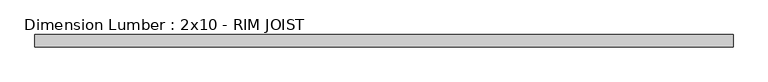
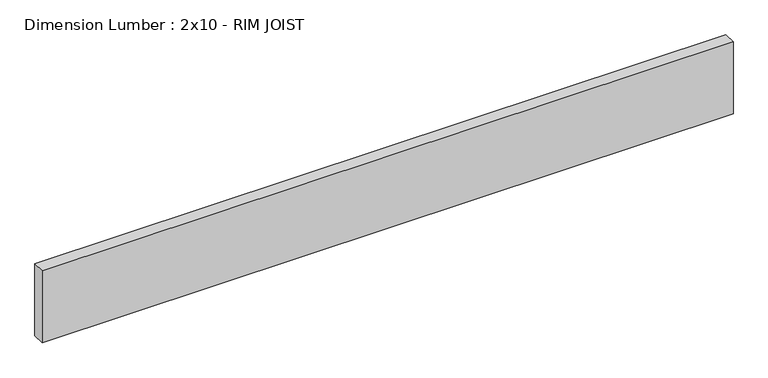
"""IFC4 building model written with IfcOpenShell, lengths in millimetres: beam geometry, Dimension Lumber : 2x10 - RIM JOIST."""

import ifcopenshell
import ifcopenshell.guid

model = None  # the IFC model being written
_history = None  # IfcOwnerHistory: only IFC2X3 demands one
_inside = {}  # id of a spatial element -> (the spatial element, [elements in it])
_under = {}  # id of a project, library or spatial element -> (it, [spatial elements below it])
_declared = {}  # id of a project -> (the project, [libraries it declares])
_typed = {}  # id of a type object -> (the type object, [elements of that type])
_made_of = {}  # id of a material, layer set ... -> (it, [elements and type objects made of it])


def new_model(schema):
    """Start an empty IFC model of exactly this schema.

    Asked for "IFC4X3", IfcOpenShell would pick the latest addendum, in which some entities
    have other attributes; the version numbers below select the first issue.
    IFC2X3 requires an IfcOwnerHistory on every rooted entity: one is made here for all.
    """
    global model, _history
    if schema == "IFC4X3":
        model = ifcopenshell.file(schema_version=(4, 3, 0, 0))
    else:
        model = ifcopenshell.file(schema=schema)
    _inside.clear()
    _under.clear()
    _declared.clear()
    _typed.clear()
    _made_of.clear()
    _history = None
    if model.schema == "IFC2X3":
        org = make("IfcOrganization", Name="unknown")
        user = make(
            "IfcPersonAndOrganization",
            ThePerson=make("IfcPerson", FamilyName="unknown"),
            TheOrganization=org,
        )
        app = make(
            "IfcApplication",
            ApplicationDeveloper=org,
            Version="unknown",
            ApplicationFullName="unknown",
            ApplicationIdentifier="unknown",
        )
        _history = make(
            "IfcOwnerHistory",
            OwningUser=user,
            OwningApplication=app,
            ChangeAction="ADDED",
            CreationDate=0,
        )
    return model


def make(cls, **values):
    """One entity of the class cls with the attributes given. An attribute that is None is left unset."""
    return model.create_entity(
        cls, **{name: value for name, value in values.items() if value is not None}
    )


def rooted(cls, **values):
    """An entity with a GlobalId (a new one), such as an element, a storey or a relation."""
    return make(cls, GlobalId=ifcopenshell.guid.new(), OwnerHistory=_history, **values)


def si_unit(unit_type, name, prefix=None):
    """IfcSIUnit, for example si_unit("LENGTHUNIT", "METRE", prefix="MILLI")."""
    return make("IfcSIUnit", UnitType=unit_type, Prefix=prefix, Name=name)


def assignment(units):
    """IfcUnitAssignment: the units of a project."""
    return None if units is None else make("IfcUnitAssignment", Units=units)


def point(xyz):
    """IfcCartesianPoint."""
    return None if xyz is None else make("IfcCartesianPoint", Coordinates=xyz)


def direction(xyz):
    """IfcDirection."""
    return None if xyz is None else make("IfcDirection", DirectionRatios=xyz)


def frame(location, z_axis=None, x_axis=None):
    """IfcAxis2Placement3D, a coordinate frame: its origin and axes. An axis left out is left unset."""
    return make(
        "IfcAxis2Placement3D",
        Location=point(location),
        Axis=direction(z_axis),
        RefDirection=direction(x_axis),
    )


def origin():
    """The frame at (0, 0, 0) with its axes left unset."""
    return frame((0.0, 0.0, 0.0))


def place(relative_to, where):
    """IfcLocalPlacement: puts the frame where relative to a parent placement (None: the world)."""
    return make(
        "IfcLocalPlacement", PlacementRelTo=relative_to, RelativePlacement=where
    )


def context(
    kind, dimensions, precision=None, world=None, true_north=None, identifier=None
):
    """IfcGeometricRepresentationContext, for example the 3D "Model" context."""
    return make(
        "IfcGeometricRepresentationContext",
        ContextIdentifier=identifier,
        ContextType=kind,
        CoordinateSpaceDimension=dimensions,
        Precision=precision,
        WorldCoordinateSystem=world,
        TrueNorth=true_north,
    )


def project(units=None, contexts=None):
    """IfcProject with its units and contexts."""
    return rooted(
        "IfcProject",
        Name="project",
        RepresentationContexts=contexts,
        UnitsInContext=assignment(units),
    )


def spatial(cls, under=None, at=None, **own):
    """A site, building, storey or space (cls), placed at a placement, below another one or the project."""
    s = rooted(cls, ObjectPlacement=at, **own)
    if under is not None:
        _under.setdefault(under.id(), (under, []))[1].append(s)
    return s


def polyline(points):
    """IfcPolyline through the points."""
    return make("IfcPolyline", Points=[point(p) for p in points])


def outline(outer, holes=None, kind="AREA"):
    """IfcArbitraryClosedProfileDef: a profile drawn as a closed curve; with holes, ...WithVoids."""
    if holes is None:
        return make("IfcArbitraryClosedProfileDef", ProfileType=kind, OuterCurve=outer)
    return make(
        "IfcArbitraryProfileDefWithVoids",
        ProfileType=kind,
        OuterCurve=outer,
        InnerCurves=holes,
    )


def extrude(swept, where, along, depth):
    """IfcExtrudedAreaSolid: the profile swept, set in the frame where, extruded along a direction by depth."""
    return make(
        "IfcExtrudedAreaSolid",
        SweptArea=swept,
        Position=where,
        ExtrudedDirection=direction(along),
        Depth=depth,
    )


def shape(context_of_items, identifier, shape_type, items):
    """IfcShapeRepresentation: the items that make up one representation, for example the "Body"."""
    return make(
        "IfcShapeRepresentation",
        ContextOfItems=context_of_items,
        RepresentationIdentifier=identifier,
        RepresentationType=shape_type,
        Items=items,
    )


def source(mapping_origin, context_of_items, identifier, shape_type, items):
    """IfcRepresentationMap: a shape defined once, which mapped items show again and again."""
    return make(
        "IfcRepresentationMap",
        MappingOrigin=mapping_origin,
        MappedRepresentation=shape(context_of_items, identifier, shape_type, items),
    )


def transform(
    local_origin,
    x_axis=None,
    y_axis=None,
    z_axis=None,
    scale=None,
    scale2=None,
    scale3=None,
    uniform=True,
):
    """IfcCartesianTransformationOperator3D, or its non-uniform kind. x_axis, y_axis, z_axis: its Axis1, 2, 3."""
    if uniform:
        return make(
            "IfcCartesianTransformationOperator3D",
            Axis1=direction(x_axis),
            Axis2=direction(y_axis),
            LocalOrigin=point(local_origin),
            Scale=scale,
            Axis3=direction(z_axis),
        )
    return make(
        "IfcCartesianTransformationOperator3DnonUniform",
        Axis1=direction(x_axis),
        Axis2=direction(y_axis),
        LocalOrigin=point(local_origin),
        Scale=scale,
        Axis3=direction(z_axis),
        Scale2=scale2,
        Scale3=scale3,
    )


def mapped(mapping_source, mapping_target):
    """IfcMappedItem: shows the shape of a source again, moved by a transform."""
    return make(
        "IfcMappedItem", MappingSource=mapping_source, MappingTarget=mapping_target
    )


def made_of(thing, what):
    """Note that an element or type object is made of a material, layer set ...; save() writes the relation."""
    if what is not None:
        _made_of.setdefault(what.id(), (what, []))[1].append(thing)
    return thing


def element(
    cls,
    number,
    at=None,
    inside=None,
    cuts=None,
    type_object=None,
    material=None,
    context=None,
    identifier="Body",
    shape_type=None,
    held_by="IfcProductDefinitionShape",
    body=None,
    shapes=None,
    **own,
):
    """One element of the class cls, such as IfcWall. Its Tag is "e" and its number.

    at: its placement. inside: the storey or other place that contains it. cuts: it is an
    opening in that element (IfcRelVoidsElement). A single representation is given by context,
    identifier, shape_type and body (its items); several are given by shapes. held_by: the class
    of the entity that holds the representations. save() writes the other relations.
    """
    e = rooted(cls, Tag="e%d" % number, ObjectPlacement=at, **own)
    if body is not None:
        shapes = [shape(context, identifier, shape_type, body)]
    if shapes is not None:
        e.Representation = make(held_by, Representations=shapes)
    if inside is not None:
        _inside.setdefault(inside.id(), (inside, []))[1].append(e)
    if cuts is not None:
        rooted(
            "IfcRelVoidsElement", RelatingBuildingElement=cuts, RelatedOpeningElement=e
        )
    if type_object is not None:
        _typed.setdefault(type_object.id(), (type_object, []))[1].append(e)
    return made_of(e, material)


def aggregate(whole, parts):
    """IfcRelAggregates: a whole, such as a stair, and the parts it consists of."""
    return rooted("IfcRelAggregates", RelatingObject=whole, RelatedObjects=parts)


def save(model, path):
    """Write the relations noted so far, then the file.

    IfcRelAggregates (storeys below a building ...), IfcRelContainedInSpatialStructure (elements
    in a storey), IfcRelDefinesByType, IfcRelAssociatesMaterial and IfcRelDeclares: one each for
    every whole, place, type object, material and project.
    """
    for whole, parts in _under.values():
        aggregate(whole, parts)
    for where, things in _inside.values():
        rooted(
            "IfcRelContainedInSpatialStructure",
            RelatedElements=things,
            RelatingStructure=where,
        )
    for kind, things in _typed.values():
        rooted("IfcRelDefinesByType", RelatedObjects=things, RelatingType=kind)
    for what, things in _made_of.values():
        rooted("IfcRelAssociatesMaterial", RelatedObjects=things, RelatingMaterial=what)
    for by, libraries in _declared.values():
        rooted("IfcRelDeclares", RelatingContext=by, RelatedDefinitions=libraries)
    model.write(path)


def dimension_lumber_2x10_rim_joist_5d972a33(model_context):
    return source(origin(), model_context, "Body", "SweptSolid", [
        extrude(outline(polyline([(1066.8, 19.05), (1066.8, -19.05), (-1066.8, -19.05), (-1066.8, 19.05), (1066.8, 19.05)])), frame((0.0, 0.0, -117.475), z_axis=(0.0, 0.0, 1.0), x_axis=(1.0, 0.0, 0.0)), (0.0, 0.0, 1.0), 234.95),
    ])


if __name__ == "__main__":
    model = new_model("IFC4")
    model_context = context("Model", 3, world=origin())
    ifc_project = project(units=[si_unit("LENGTHUNIT", "METRE", prefix="MILLI")], contexts=[model_context])
    site = spatial("IfcSite", under=ifc_project)
    building = spatial("IfcBuilding", under=site)
    placement = place(None, origin())
    dimension_lumber_2x10_rim_joist_shape = dimension_lumber_2x10_rim_joist_5d972a33(model_context)
    element("IfcBeam", 1, ObjectType="Dimension Lumber : 2x10 - RIM JOIST", at=placement, inside=building, context=model_context, shape_type="MappedRepresentation", body=[
        mapped(dimension_lumber_2x10_rim_joist_shape, transform((0.0, 0.0, 0.0), x_axis=(1.0, 0.0, 0.0), y_axis=(0.0, 1.0, 0.0), z_axis=(0.0, 0.0, 1.0))),
    ])
    save(model, "model.ifc")

# Revit data of these elements
# Type "Dimension Lumber : 2x10 - RIM JOIST"
#   Assembly Code = "B10"
#   A = 0.0963889 SF
#   Length [instance default] = 5' - 0"
#   b = 0' - 1 1/2"
#   d = 0' - 9 1/4"
#   Structural Material = TREATED 2X10 RIM JOIST
# Element 1 (IfcBeam, "Dimension Lumber : 2x10 - RIM JOIST")
#   Materials on its faces: "TREATED 2X10 RIM JOIST"
# Materials
#   "TREATED 2X10 RIM JOIST": class "Wood", colour RGB 234 198 147, transparency 0, Description = "Pinus Echinata", Cost = 0
